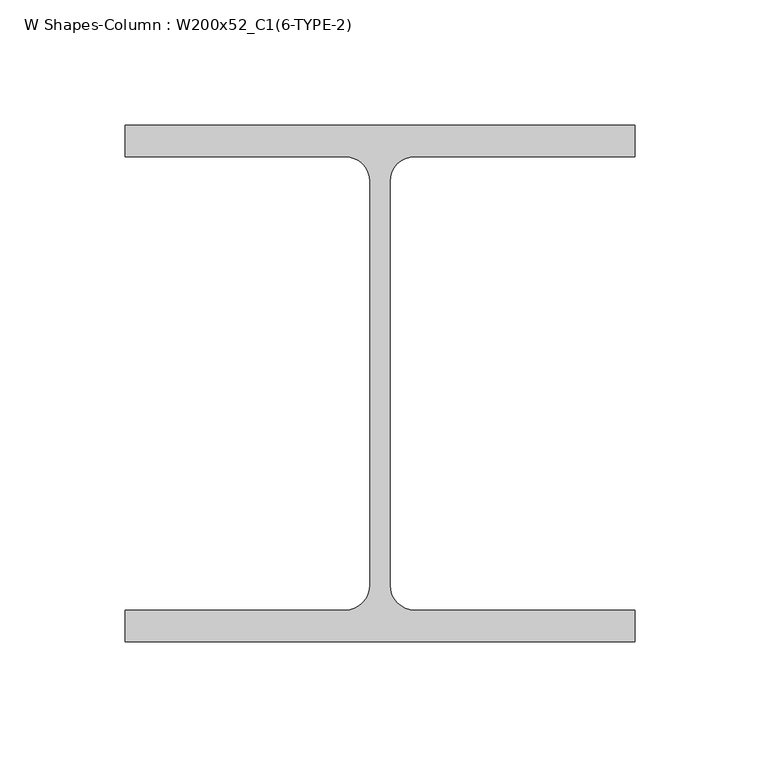
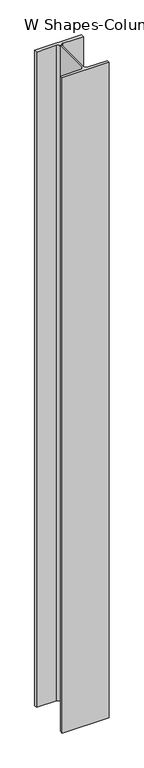
"""IFC4 building model written with IfcOpenShell, lengths in millimetres: column geometry, W Shapes-Column : W200x52_C1(6-TYPE-2)."""

from ifc_helpers import new_model, si_unit, point, frame, frame_2d, origin, place, context, project, spatial, polyline, circle_curve, trimmed, segment, composite_curve, outline, extrude, source, transform, mapped, element, save


def w_shapes_column_w200x52_c1_6_type_2_2bcbd5a8(model_context):
    return source(origin(), model_context, "Body", "SweptSolid", [
        extrude(outline(composite_curve([segment(polyline([(101.854, 103.124), (101.854, 90.551), (13.9446, 90.551)]), True, "CONTINUOUS"), segment(trimmed(circle_curve(frame_2d((13.9446, 80.5434)), 10.0076), [point((13.9446, 90.551))], [point((3.937, 80.5434))], True, "CARTESIAN"), True, "CONTINUOUS"), segment(polyline([(3.937, 80.5434), (3.937, -80.5434)]), True, "CONTINUOUS"), segment(trimmed(circle_curve(frame_2d((13.9446, -80.5434)), 10.0076), [point((3.937, -80.5434))], [point((13.9446, -90.551))], True, "CARTESIAN"), True, "CONTINUOUS"), segment(polyline([(13.9446, -90.551), (101.854, -90.551), (101.854, -103.124), (-101.854, -103.124), (-101.854, -90.551), (-13.9446, -90.551)]), True, "CONTINUOUS"), segment(trimmed(circle_curve(frame_2d((-13.9446, -80.5434)), 10.0076), [point((-13.9446, -90.551))], [point((-3.937, -80.5434))], True, "CARTESIAN"), True, "CONTINUOUS"), segment(polyline([(-3.937, -80.5434), (-3.937, 80.5434)]), True, "CONTINUOUS"), segment(trimmed(circle_curve(frame_2d((-13.9446, 80.5434)), 10.0076), [point((-3.937, 80.5434))], [point((-13.9446, 90.551))], True, "CARTESIAN"), True, "CONTINUOUS"), segment(polyline([(-13.9446, 90.551), (-101.854, 90.551), (-101.854, 103.124), (101.854, 103.124)]), True, "CONTINUOUS")], self_intersect=False)), frame((0.0, 0.0, 200.0), z_axis=(0.0, 0.0, 1.0), x_axis=(1.0, 0.0, 0.0)), (0.0, 0.0, 1.0), 3000.0),
    ])


if __name__ == "__main__":
    model = new_model("IFC4")
    model_context = context("Model", 3, world=origin())
    ifc_project = project(units=[si_unit("LENGTHUNIT", "METRE", prefix="MILLI")], contexts=[model_context])
    site = spatial("IfcSite", under=ifc_project)
    building = spatial("IfcBuilding", under=site)
    placement = place(None, origin())
    w_shapes_column_w200x52_c1_6_type_2_shape = w_shapes_column_w200x52_c1_6_type_2_2bcbd5a8(model_context)
    element("IfcColumn", 1, ObjectType="W Shapes-Column : W200x52_C1(6-TYPE-2)", at=placement, inside=building, context=model_context, shape_type="MappedRepresentation", body=[
        mapped(w_shapes_column_w200x52_c1_6_type_2_shape, transform((0.0, 0.0, 0.0), x_axis=(1.0, 0.0, 0.0), y_axis=(0.0, 1.0, 0.0), z_axis=(0.0, 0.0, 1.0))),
    ])
    save(model, "model.ifc")

# Revit data of these elements
# Type "W Shapes-Column : W200x52_C1(6-TYPE-2)"
#   Section Name Key = "W8X35"
#   Assembly Code = "B10"
#   Width = 20.3708 cm
#   Web Thickness = 0.7874 cm
#   Web Fillet = 1.0008 cm
#   Warping Constant = 166223.7 cm⁶
#   Torsional Moment of Inertia = 32.0082 cm⁴
#   Section Area = 66.4515 cm²
#   Plastic Modulus weak axis = 263.832 cm³
#   Plastic Modulus strong axis = 568.631 cm³
#   Perimeter = 1.1936 m²/m
#   Nominal Weight = 52.0857 kgf/m
#   Moment of Inertia weak axis = 1773.15 cm⁴
#   Moment of Inertia strong axis = 5286.14 cm⁴
#   Height = 20.6248 cm
#   Flange Thickness = 1.2573 cm
#   Elastic Modulus weak axis = 173.703 cm³
#   Elastic Modulus strong axis = 511.276 cm³
#   Clear Web Height = 14.605 cm
#   Centroid Vertical = 10.3124 cm
#   Centroid Horizontal = 10.1854 cm
#   Bolt Spacing = 13.97 cm
#   Structural Material [instance default] = Steel ASTM A992
#   Principal Axes Angle = 0
# Element 1 (IfcColumn, "W Shapes-Column : W200x52_C1(6-TYPE-2)")
#   Structural Material = none
# Materials
#   "Steel ASTM A992": class "Metal", colour RGB 199 199 199, transparency 0, Description = "Structural steel 50ksi", Cost = 0
